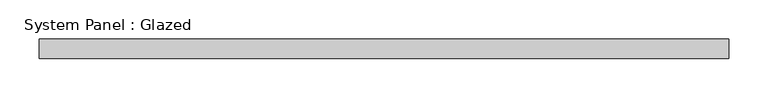
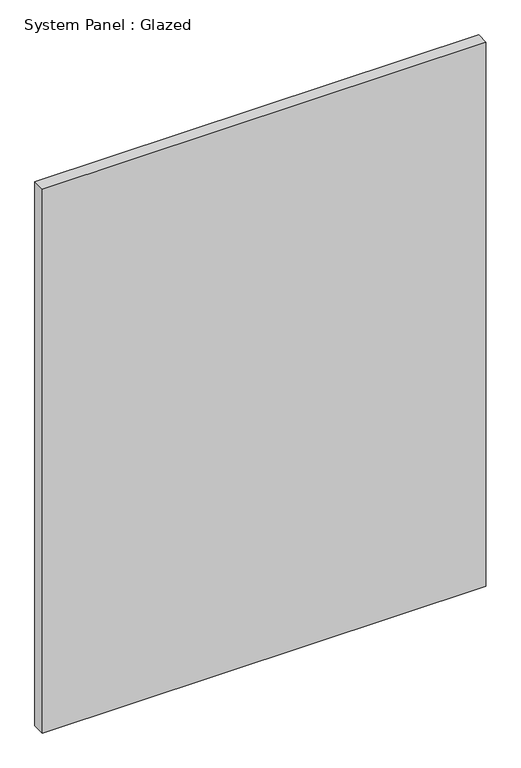
"""IFC4 building model written with IfcOpenShell, lengths in millimetres: plate geometry, System Panel : Glazed."""

from ifc_helpers import new_model, si_unit, origin, origin_with_axes, place, context, project, spatial, polyline, outline, extrude, source, transform, mapped, element, save


def system_panel_glazed_eb4afb5f(model_context):
    return source(origin(), model_context, "Body", "SweptSolid", [
        extrude(outline(polyline([(440.8714287, -12.7), (-440.8714287, -12.7), (-440.8714287, 12.7), (440.8714287, 12.7), (440.8714287, -12.7)])), origin_with_axes(), (0.0, 0.0, 1.0), 1143.0),
    ])


if __name__ == "__main__":
    model = new_model("IFC4")
    model_context = context("Model", 3, world=origin())
    ifc_project = project(units=[si_unit("LENGTHUNIT", "METRE", prefix="MILLI")], contexts=[model_context])
    site = spatial("IfcSite", under=ifc_project)
    building = spatial("IfcBuilding", under=site)
    placement = place(None, origin())
    system_panel_glazed_shape = system_panel_glazed_eb4afb5f(model_context)
    element("IfcPlate", 1, ObjectType="System Panel : Glazed", at=placement, inside=building, context=model_context, shape_type="MappedRepresentation", body=[
        mapped(system_panel_glazed_shape, transform((0.0, 0.0, 0.0), x_axis=(1.0, 0.0, 0.0), y_axis=(0.0, 1.0, 0.0), z_axis=(0.0, 0.0, 1.0))),
    ])
    save(model, "model.ifc")

# Revit data of these elements
# Element 1 (IfcPlate, "System Panel : Glazed")
#   Materials on its faces: "Glass"
# Materials
#   "Glass": class "Glass", colour RGB 218 227 224, transparency 0.85, Description = "Soda Lime Glass", Cost = 0
